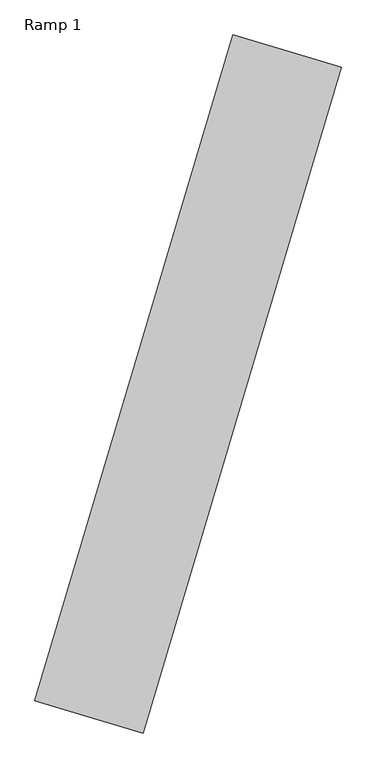
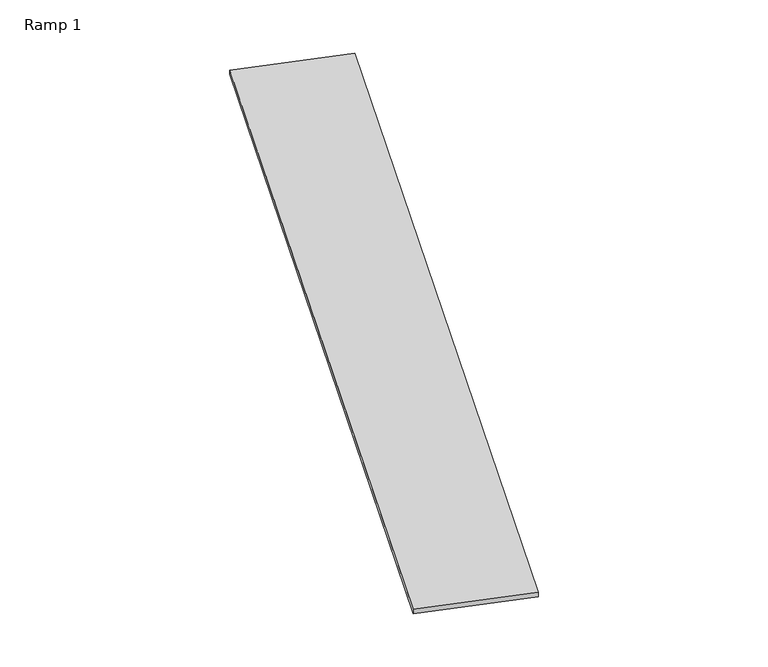
"""IFC4 building model written with IfcOpenShell, lengths in millimetres: ramp geometry, Ramp 1."""

from ifc_helpers import new_model, si_unit, frame, origin, place, context, project, spatial, polyline, outline, extrude, source, transform, mapped, element, save


def ramp_1_e6d8d0b2(model_context):
    return source(origin(), model_context, "Body", "SweptSolid", [
        extrude(outline(polyline([(-4700.0, -30704.1914312), (0.0, 0.0), (202.3295842, 0.0), (-4497.6704158, -30704.1914312), (-4700.0, -30704.1914312)])), frame((38391.793903, 120222.1050221, 5300.0), z_axis=(-0.9584455062260432, 0.28527567648697966, 0.0), x_axis=(0.0, 0.0, -1.0)), (0.0, 0.0, 1.0), 5000.0),
    ])


if __name__ == "__main__":
    model = new_model("IFC4")
    model_context = context("Model", 3, world=origin())
    ifc_project = project(units=[si_unit("LENGTHUNIT", "METRE", prefix="MILLI")], contexts=[model_context])
    site = spatial("IfcSite", under=ifc_project)
    building = spatial("IfcBuilding", under=site)
    placement = place(None, origin())
    ramp_1_shape = ramp_1_e6d8d0b2(model_context)
    element("IfcRamp", 1, ObjectType="Ramp 1", at=placement, inside=building, context=model_context, shape_type="MappedRepresentation", body=[
        mapped(ramp_1_shape, transform((0.0, 0.0, 0.0), x_axis=(1.0, 0.0, 0.0), y_axis=(0.0, 1.0, 0.0), z_axis=(0.0, 0.0, 1.0))),
    ])
    save(model, "model.ifc")
